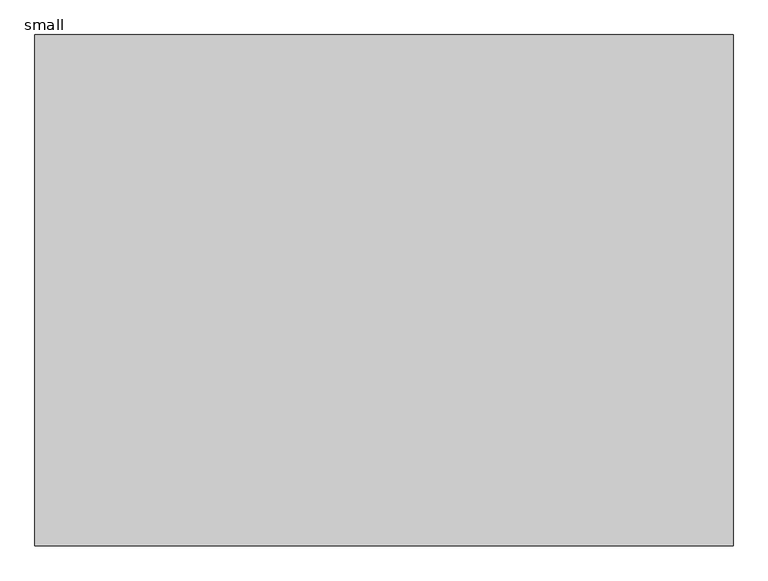
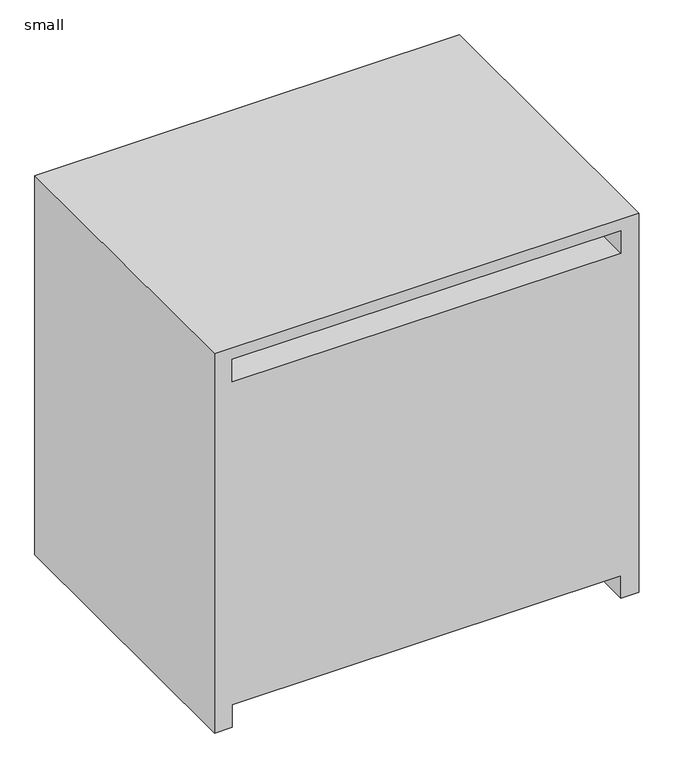
"""IFC4 building model written with IfcOpenShell, lengths in millimetres: proxy geometry, 261200 - Medium-Voltage Transformers - Generic : small."""

from ifc_helpers import new_model, si_unit, frame, origin, place, context, project, spatial, polyline, outline, extrude, source, transform, mapped, element, save


def small_32f65543(model_context):
    return source(origin(), model_context, "Body", "SweptSolid", [
        extrude(outline(polyline([(1701.8, 901.7), (1701.8, -901.7), (0.0, -901.7), (0.0, -825.5), (101.6, -825.5), (101.6, 825.5), (0.0, 825.5), (0.0, 901.7), (1701.8, 901.7)]), holes=[polyline([(1651.0, 825.5), (1549.4, 825.5), (1549.4, -825.5), (1651.0, -825.5), (1651.0, 825.5)])]), frame((0.0, -660.4, 0.0), z_axis=(0.0, 1.0, 0.0), x_axis=(0.0, 0.0, 1.0)), (0.0, 0.0, 1.0), 1320.8),
    ])


if __name__ == "__main__":
    model = new_model("IFC4")
    model_context = context("Model", 3, world=origin())
    ifc_project = project(units=[si_unit("LENGTHUNIT", "METRE", prefix="MILLI")], contexts=[model_context])
    site = spatial("IfcSite", under=ifc_project)
    building = spatial("IfcBuilding", under=site)
    placement = place(None, origin())
    small_shape = small_32f65543(model_context)
    element("IfcBuildingElementProxy", 1, Name="261200 - Medium-Voltage Transformers - Generic : small", ObjectType="261200 - Medium-Voltage Transformers - Generic : small", at=placement, inside=building, context=model_context, shape_type="MappedRepresentation", body=[
        mapped(small_shape, transform((0.0, 0.0, 0.0), x_axis=(1.0, 0.0, 0.0), y_axis=(0.0, 1.0, 0.0), z_axis=(0.0, 0.0, 1.0))),
    ])
    save(model, "model.ifc")

# Revit data of these elements
# Type "261200 - Medium-Voltage Transformers - Generic : small"
#   Weight = "5500"
#   Wattage = "DO NOT USE"
#   Voltage = "DO NOT USE"
#   URL = "http://www.usa.siemens.com/ce"
#   Transformer Material = "Aluminum"
#   Product Page URL = "http://www.sea.siemens.com/us/Products/PowerDistribution/Product/Transformers/Pages/Transformers.aspx"
#   Product Documentation Link = "http://www.sea.siemens.com/us/internet-dms/Internet/ConsultingEngineersComm/General/Docs/drytrans.pdf"
#   Model = "3F3Y015K13TP1"
#   Manufacturer = "Siemens Industry"
#   KVA = "750"
#   K Factor = "13"
#   Description = "Transformer"
#   Deg Rise = "150"
#   Copyright © = "© Siemens Industry, Inc. 2011"
#   CTRL Connector Description = "Equipment Power"
#   BOM URL [instance default] = ""
#   Assembly Code = "D5090900"
#   clearance = 3' - 0"
#   Width = 5' - 11"
#   Primary Voltage = 480 V
#   Power Factor = 1
#   Height = 5' - 7"
#   Depth = 4' - 4"
#   Apparent Load [instance default] = 0 VA
#   Has Not Contacted Siemens For Configuration [instance default] = no
#   Contacted Siemens For Configuration [instance default] = yes
#   Text Material = Paint- Siemens - Dark
#   Frame Material = ELECTRICAL TRANSFORMERS
# Element 1 (IfcBuildingElementProxy, "261200 - Medium-Voltage Transformers - Generic : small")
#   Materials on its faces: "ELECTRICAL TRANSFORMERS"
# Materials
#   "Paint- Siemens - Dark": class "Metal", colour RGB 175 38 68, transparency 0
#   "ELECTRICAL TRANSFORMERS": class "Metal", colour RGB 63 114 97, transparency 0, Cost = 0
